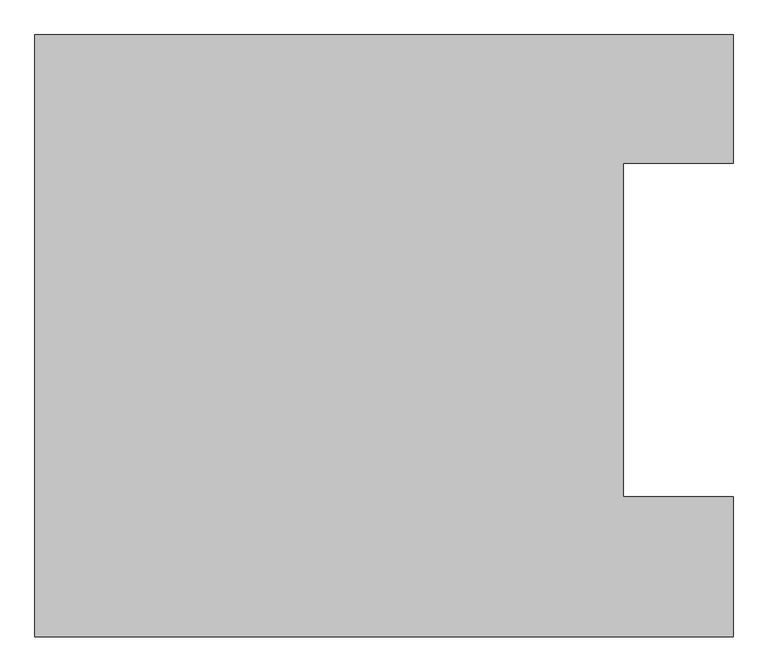
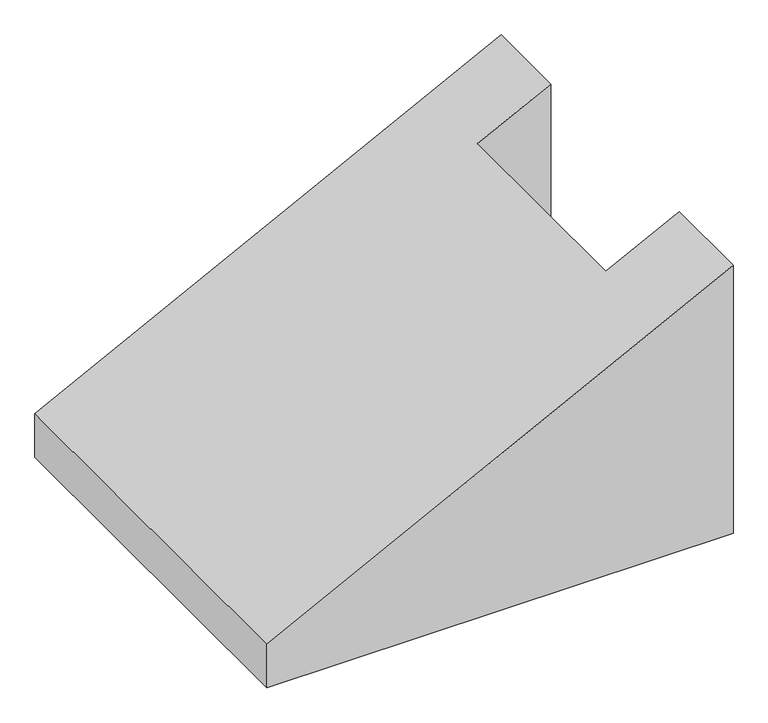
"""IFC4 building model written with IfcOpenShell, lengths in millimetres: proxy geometry, 0_3d."""

from ifc_helpers import new_model, si_unit, origin, place, context, project, spatial, faceted_brep, source, transform, mapped, element, save


def generic_models_e2c044ad(model_context):
    return source(origin(), model_context, "Body", "Brep", [
        faceted_brep([(5495.0, 4420.0, 3438.4620158), (6520.0, 4420.0, 3960.7256015), (6520.0, 5620.0, 3960.7256015), (0.0, 5620.0, 638.6196708), (0.0, 0.0, 638.6196708), (6520.0, 0.0, 3960.7256015), (6520.0, 1305.0, 3960.7256015), (5495.0, 1305.0, 3438.4620158), (0.0, 0.0, 0.0), (6520.0, 0.0, 0.0), (0.0, 5620.0, 0.0), (6520.0, 5620.0, 0.0), (5495.0, 4420.0, 0.0), (6520.0, 4420.0, 0.0), (5495.0, 1305.0, 0.0), (6520.0, 1305.0, 0.0)], [[[0, 1, 2, 3, 4, 5, 6, 7]], [[5, 4, 8, 9]], [[4, 3, 10, 8]], [[3, 2, 11, 10]], [[1, 0, 12, 13]], [[0, 7, 14, 12]], [[7, 6, 15, 14]], [[9, 15, 6, 5]], [[13, 11, 2, 1]], [[11, 13, 12, 14, 15, 9, 8, 10]]]),
    ])


if __name__ == "__main__":
    model = new_model("IFC4")
    model_context = context("Model", 3, world=origin())
    ifc_project = project(units=[si_unit("LENGTHUNIT", "METRE", prefix="MILLI")], contexts=[model_context])
    site = spatial("IfcSite", under=ifc_project)
    building = spatial("IfcBuilding", under=site)
    placement = place(None, origin())
    generic_models_shape = generic_models_e2c044ad(model_context)
    element("IfcBuildingElementProxy", 1, Name="0_3d", ObjectType="0_3d", at=placement, inside=building, context=model_context, shape_type="MappedRepresentation", body=[
        mapped(generic_models_shape, transform((0.0, 0.0, 0.0), x_axis=(1.0, 0.0, 0.0), y_axis=(0.0, 1.0, 0.0), z_axis=(0.0, 0.0, 1.0))),
    ])
    save(model, "model.ifc")

# Revit data of these elements
# Element 1 (IfcBuildingElementProxy, "0_3d")
#   Materials on its faces: "*1"
# Materials
#   "*1": class "Unassigned", colour RGB 175 175 175, transparency 0
